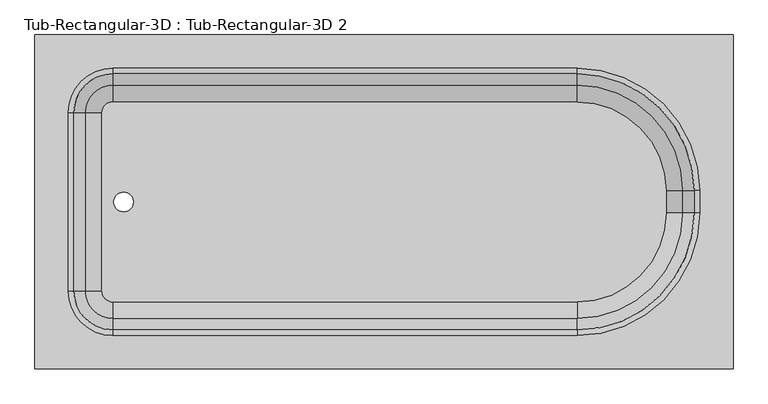
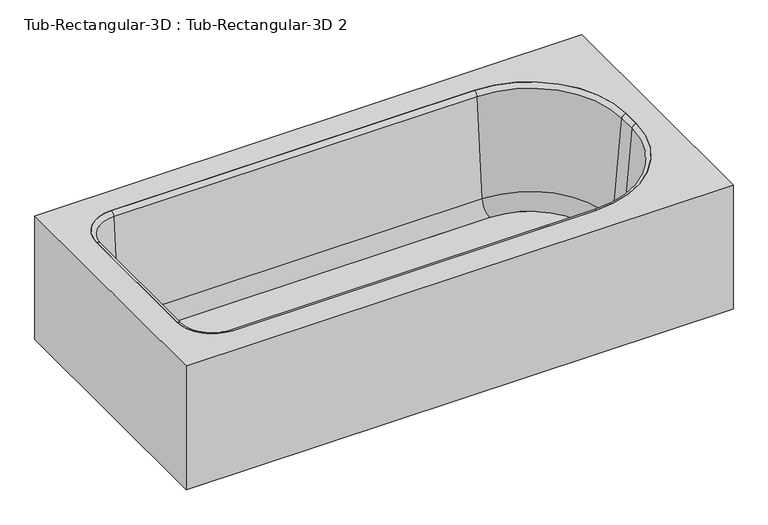
"""IFC4 building model written with IfcOpenShell, lengths in millimetres: flow terminal geometry, Tub-Rectangular-3D : Tub-Rectangular-3D 2."""

from ifc_helpers import new_model, si_unit, point, frame, frame_2d, origin, place, context, project, spatial, polyline, circle_curve, ellipse_curve, trimmed, segment, composite_curve, outline, extrude, source, transform, mapped, element, save
from ifc_brep_helpers import plane_surface, cylinder_surface, revolved_surface, advanced_brep


def tub_rectangular_3d_tub_rectangular_3d_2_b18e5bc2(model_context):
    return source(origin(), model_context, "Body", "SolidModel", [
        advanced_brep(
        [(480.0720313, 830.2625, 381.0), (-1110.6029687, 830.2625, 381.0), (-1110.6029687, 68.2625, 381.0), (480.0720313, 68.2625, 381.0), (-932.8029687, 754.0625, 381.0), (124.4720313, 754.0625, 381.0), (403.8720313, 474.6625, 381.0), (403.8720313, 423.8625, 381.0), (124.4720313, 144.4625, 381.0), (-932.8029687, 144.4625, 381.0), (-1034.4029687, 246.0625, 381.0), (-1034.4029687, 652.4625, 381.0), (461.0220313, 811.2125, 361.95), (461.0220313, 87.3125, 361.95), (-1091.5529687, 87.3125, 361.95), (-1091.5529687, 811.2125, 361.95), (-932.8029687, 754.0625, 361.95), (-1034.4029687, 652.4625, 361.95), (-1034.4029687, 246.0625, 361.95), (-932.8029687, 144.4625, 361.95), (124.4720313, 144.4625, 361.95), (403.8720313, 423.8625, 361.95), (403.8720313, 474.6625, 361.95), (124.4720313, 754.0625, 361.95), (480.0720313, 830.2625, 0.0), (-1110.6029687, 830.2625, 0.0), (-1110.6029687, 68.2625, 0.0), (480.0720313, 68.2625, 0.0), (461.0220313, 811.2125, 0.0), (-1091.5529687, 811.2125, 0.0), (-1091.5529687, 87.3125, 0.0), (461.0220313, 87.3125, 0.0)],
        [
            (0, 1),
            (1, 2),
            (2, 3),
            (3, 0),
            (4, 5),
            (5, 6, circle_curve(frame((124.4720313, 474.6625, 381.0), z_axis=(0.0, 0.0, -1.0), x_axis=(0.0, 1.0, 0.0)), 279.4)),
            (6, 7),
            (7, 8, circle_curve(frame((124.4720313, 423.8625, 381.0), z_axis=(0.0, 0.0, -1.0), x_axis=(0.0, 1.0, 0.0)), 279.4)),
            (8, 9),
            (9, 10, circle_curve(frame((-932.8029687, 246.0625, 381.0), z_axis=(0.0, 0.0, -1.0), x_axis=(0.0, 1.0, 0.0)), 101.6)),
            (10, 11),
            (11, 4, circle_curve(frame((-932.8029687, 652.4625, 381.0), z_axis=(0.0, 0.0, -1.0), x_axis=(0.0, 1.0, 0.0)), 101.6)),
            (12, 13),
            (13, 14),
            (14, 15),
            (15, 12),
            (16, 17, circle_curve(frame((-932.8029687, 652.4625, 361.95), z_axis=(0.0, 0.0, 1.0), x_axis=(0.0, 1.0, 0.0)), 101.6)),
            (17, 18),
            (18, 19, circle_curve(frame((-932.8029687, 246.0625, 361.95), z_axis=(0.0, 0.0, 1.0), x_axis=(0.0, 1.0, 0.0)), 101.6)),
            (19, 20),
            (20, 21, circle_curve(frame((124.4720313, 423.8625, 361.95), z_axis=(0.0, 0.0, 1.0), x_axis=(0.0, 1.0, 0.0)), 279.4)),
            (21, 22),
            (22, 23, circle_curve(frame((124.4720313, 474.6625, 361.95), z_axis=(0.0, 0.0, 1.0), x_axis=(0.0, 1.0, 0.0)), 279.4)),
            (23, 16),
            (0, 24),
            (24, 25),
            (25, 1),
            (25, 26),
            (26, 2),
            (26, 27),
            (27, 3),
            (27, 24),
            (4, 16),
            (23, 5),
            (22, 6),
            (21, 7),
            (20, 8),
            (19, 9),
            (18, 10),
            (17, 11),
            (28, 29),
            (29, 30),
            (30, 31),
            (31, 28),
            (31, 13),
            (12, 28),
            (30, 14),
            (29, 15),
        ],
        [
            plane_surface(frame((-1110.6029687, 830.2625, 381.0), z_axis=(0.0, 0.0, 1.0), x_axis=(-1.0, 0.0, 0.0))),
            plane_surface(frame((-1110.6029687, 830.2625, 361.95), z_axis=(0.0, 0.0, -1.0), x_axis=(1.0, 0.0, 0.0))),
            plane_surface(frame((480.0720313, 830.2625, 381.0), z_axis=(0.0, 1.0, 0.0), x_axis=(0.0, 0.0, -1.0))),
            plane_surface(frame((-1110.6029687, 830.2625, 381.0), z_axis=(-1.0, 0.0, 0.0), x_axis=(0.0, 0.0, -1.0))),
            plane_surface(frame((-1110.6029687, 68.2625, 381.0), z_axis=(0.0, -1.0, 0.0), x_axis=(0.0, 0.0, -1.0))),
            plane_surface(frame((480.0720313, 68.2625, 381.0), z_axis=(1.0, 0.0, 0.0), x_axis=(0.0, 0.0, -1.0))),
            plane_surface(frame((-932.8029687, 754.0625, 381.0), z_axis=(0.0, -1.0, 0.0), x_axis=(0.0, 0.0, -1.0))),
            revolved_surface(polyline([(124.4720313, 754.0625, 361.95), (124.4720313, 754.0625, 381.0)]), (124.4720313, 474.6625, 381.0), (0.0, 0.0, -1.0)),
            plane_surface(frame((403.8720313, 474.6625, 381.0), z_axis=(-1.0, 0.0, 0.0), x_axis=(0.0, 0.0, -1.0))),
            revolved_surface(polyline([(124.4720313, 703.2625, 361.95), (124.4720313, 703.2625, 381.0)]), (124.4720313, 423.8625, 381.0), (0.0, 0.0, -1.0)),
            plane_surface(frame((124.4720313, 144.4625, 381.0), z_axis=(0.0, 1.0, 0.0), x_axis=(0.0, 0.0, -1.0))),
            revolved_surface(polyline([(-932.8029687, 347.6625, 361.95), (-932.8029687, 347.6625, 381.0)]), (-932.8029687, 246.0625, 381.0), (0.0, 0.0, -1.0)),
            plane_surface(frame((-1034.4029687, 246.0625, 381.0), z_axis=(1.0, 0.0, 0.0), x_axis=(0.0, 0.0, -1.0))),
            revolved_surface(polyline([(-932.8029687, 754.0625, 361.95), (-932.8029687, 754.0625, 381.0)]), (-932.8029687, 652.4625, 381.0), (0.0, 0.0, -1.0)),
            plane_surface(frame((-1110.6029687, 830.2625, 0.0), z_axis=(0.0, 0.0, -1.0), x_axis=(1.0, 0.0, 0.0))),
            plane_surface(frame((461.0220313, 811.2125, 361.95), z_axis=(-1.0, 0.0, 0.0), x_axis=(0.0, 0.0, -1.0))),
            plane_surface(frame((461.0220313, 87.3125, 361.95), z_axis=(0.0, 1.0, 0.0), x_axis=(0.0, 0.0, -1.0))),
            plane_surface(frame((-1091.5529687, 87.3125, 361.95), z_axis=(1.0, 0.0, 0.0), x_axis=(0.0, 0.0, -1.0))),
            plane_surface(frame((-1091.5529687, 811.2125, 361.95), z_axis=(0.0, -1.0, 0.0), x_axis=(0.0, 0.0, -1.0))),
        ],
        [
            (0, [[1, 2, 3, 4], [5, 6, 7, 8, 9, 10, 11, 12]]),
            (1, [[13, 14, 15, 16], [17, 18, 19, 20, 21, 22, 23, 24]]),
            (2, [[-1, 25, 26, 27]]),
            (3, [[-2, -27, 28, 29]]),
            (4, [[-3, -29, 30, 31]]),
            (5, [[-25, -4, -31, 32]]),
            (6, [[-5, 33, -24, 34]]),
            (7, [[-6, -34, -23, 35]]),
            (8, [[-7, -35, -22, 36]]),
            (9, [[-8, -36, -21, 37]]),
            (10, [[-9, -37, -20, 38]]),
            (11, [[-10, -38, -19, 39]]),
            (12, [[-11, -39, -18, 40]]),
            (13, [[-12, -40, -17, -33]]),
            (14, [[-32, -30, -28, -26], [41, 42, 43, 44]]),
            (15, [[-44, 45, -13, 46]]),
            (16, [[-43, 47, -14, -45]]),
            (17, [[-42, 48, -15, -47]]),
            (18, [[-41, -46, -16, -48]]),
        ],
    ),
        extrude(outline(composite_curve([segment(trimmed(circle_curve(frame_2d((124.4720313, 474.6625)), 202.7964741), [point((124.4720313, 677.4589741))], [point((327.2685054, 474.6625))], False, "CARTESIAN"), True, "CONTINUOUS"), segment(polyline([(327.2685054, 474.6625), (327.2685054, 423.8625)]), True, "CONTINUOUS"), segment(trimmed(circle_curve(frame_2d((124.4720313, 423.8625)), 202.7964741), [point((327.2685054, 423.8625))], [point((124.4720313, 221.0660259))], False, "CARTESIAN"), True, "CONTINUOUS"), segment(polyline([(124.4720313, 221.0660259), (-932.8029687, 221.0660259)]), True, "CONTINUOUS"), segment(trimmed(circle_curve(frame_2d((-932.8029687, 246.0625)), 24.9964741), [point((-932.8029687, 221.0660259))], [point((-957.7994428, 246.0625))], False, "CARTESIAN"), True, "CONTINUOUS"), segment(polyline([(-957.7994428, 246.0625), (-957.7994428, 652.4625)]), True, "CONTINUOUS"), segment(trimmed(circle_curve(frame_2d((-932.8029687, 652.4625)), 24.9964741), [point((-957.7994428, 652.4625))], [point((-932.8029687, 677.4589741))], False, "CARTESIAN"), True, "CONTINUOUS"), segment(polyline([(-932.8029687, 677.4589741), (124.4720313, 677.4589741)]), True, "CONTINUOUS")], self_intersect=False), holes=[composite_curve([segment(trimmed(circle_curve(frame_2d((-908.510206, 449.2625)), 22.225), [point((-908.510206, 471.4875))], [point((-908.510206, 427.0375))], True, "CARTESIAN"), True, "CONTINUOUS"), segment(trimmed(circle_curve(frame_2d((-908.510206, 449.2625)), 22.225), [point((-908.510206, 427.0375))], [point((-908.510206, 471.4875))], True, "CARTESIAN"), True, "CONTINUOUS")], self_intersect=False)]), frame((0.0, 0.0, 16.863573), z_axis=(0.0, 0.0, 1.0), x_axis=(1.0, 0.0, 0.0)), (0.0, 0.0, 1.0), 19.05),
        advanced_brep(
        [(-995.7544608, 652.4625, 70.6929392), (-932.8029687, 715.4139921, 70.6929392), (-932.8029687, 741.5845035, 369.8232535), (-1021.9249722, 652.4625, 369.8232535), (-957.7994428, 652.4625, 35.913573), (-932.8029687, 677.4589741, 35.913573), (-957.7994428, 652.4625, 16.863573), (-932.8029687, 677.4589741, 16.863573), (-1034.4029687, 652.4625, 16.863573), (-932.8029687, 754.0625, 16.863573), (-1034.4029687, 652.4625, 381.0), (-932.8029687, 754.0625, 381.0), (-1021.9249722, 246.0625, 369.8232535), (-995.7544608, 246.0625, 70.6929392), (-957.7994428, 246.0625, 35.913573), (-957.7994428, 246.0625, 16.863573), (-1034.4029687, 246.0625, 16.863573), (-1034.4029687, 246.0625, 381.0), (-932.8029687, 183.1110079, 70.6929392), (-932.8029687, 156.9404965, 369.8232535), (-932.8029687, 221.0660259, 35.913573), (-932.8029687, 221.0660259, 16.863573), (-932.8029687, 144.4625, 16.863573), (-932.8029687, 144.4625, 381.0), (124.4720313, 156.9404965, 369.8232535), (124.4720313, 183.1110079, 70.6929392), (124.4720313, 221.0660259, 35.913573), (124.4720313, 221.0660259, 16.863573), (124.4720313, 144.4625, 16.863573), (124.4720313, 144.4625, 381.0), (365.2235234, 423.8625, 70.6929392), (391.3940348, 423.8625, 369.8232535), (327.2685054, 423.8625, 35.913573), (327.2685054, 423.8625, 16.863573), (403.8720313, 423.8625, 16.863573), (403.8720313, 423.8625, 381.0), (391.3940348, 474.6625, 369.8232535), (365.2235234, 474.6625, 70.6929392), (327.2685054, 474.6625, 35.913573), (327.2685054, 474.6625, 16.863573), (403.8720313, 474.6625, 16.863573), (403.8720313, 474.6625, 381.0), (124.4720313, 715.4139921, 70.6929392), (124.4720313, 741.5845035, 369.8232535), (124.4720313, 677.4589741, 35.913573), (124.4720313, 677.4589741, 16.863573), (124.4720313, 754.0625, 16.863573), (124.4720313, 754.0625, 381.0)],
        [
            (0, 1, circle_curve(frame((-932.8029687, 652.4625, 70.6929392), z_axis=(0.0, 0.0, -1.0), x_axis=(0.0, 1.0, 0.0)), 62.9514921)),
            (1, 2),
            (2, 3, circle_curve(frame((-932.8029687, 652.4625, 369.8232535), z_axis=(0.0, 0.0, 1.0), x_axis=(0.0, 1.0, 0.0)), 89.1220035)),
            (3, 0),
            (4, 5, circle_curve(frame((-932.8029687, 652.4625, 35.913573), z_axis=(0.0, 0.0, -1.0), x_axis=(0.0, 1.0, 0.0)), 24.9964741)),
            (5, 1, circle_curve(frame((-932.8029687, 677.4589741, 74.013573), z_axis=(1.0, 0.0, 0.0), x_axis=(0.0, -1.0, 0.0)), 38.1)),
            (0, 4, circle_curve(frame((-957.7994428, 652.4625, 74.013573), z_axis=(0.0, -1.0, 0.0), x_axis=(1.0, 0.0, 0.0)), 38.1)),
            (6, 7, circle_curve(frame((-932.8029687, 652.4625, 16.863573), z_axis=(0.0, 0.0, -1.0), x_axis=(0.0, 1.0, 0.0)), 24.9964741)),
            (7, 5),
            (4, 6),
            (8, 9, circle_curve(frame((-932.8029687, 652.4625, 16.863573), z_axis=(0.0, 0.0, -1.0), x_axis=(0.0, 1.0, 0.0)), 101.6)),
            (9, 7),
            (6, 8),
            (10, 11, circle_curve(frame((-932.8029687, 652.4625, 381.0), z_axis=(0.0, 0.0, -1.0), x_axis=(0.0, 1.0, 0.0)), 101.6)),
            (11, 9),
            (8, 10),
            (2, 11, circle_curve(frame((-932.8029687, 754.0625, 368.4462547), z_axis=(-1.0, 0.0, 0.0), x_axis=(0.0, -1.0, 0.0)), 12.5537453)),
            (10, 3, circle_curve(frame((-1034.4029687, 652.4625, 368.4462547), z_axis=(0.0, 1.0, 0.0), x_axis=(1.0, 0.0, 0.0)), 12.5537453)),
            (3, 12),
            (12, 13),
            (13, 0),
            (13, 14, circle_curve(frame((-957.7994428, 246.0625, 74.013573), z_axis=(0.0, -1.0, 0.0), x_axis=(1.0, 0.0, 0.0)), 38.1)),
            (14, 4),
            (14, 15),
            (15, 6),
            (15, 16),
            (16, 8),
            (16, 17),
            (17, 10),
            (17, 12, circle_curve(frame((-1034.4029687, 246.0625, 368.4462547), z_axis=(0.0, 1.0, 0.0), x_axis=(1.0, 0.0, 0.0)), 12.5537453)),
            (18, 13, circle_curve(frame((-932.8029687, 246.0625, 70.6929392), z_axis=(0.0, 0.0, -1.0), x_axis=(-1.0, 0.0, 0.0)), 62.9514921)),
            (12, 19, circle_curve(frame((-932.8029687, 246.0625, 369.8232535), z_axis=(0.0, 0.0, 1.0), x_axis=(-1.0, 0.0, 0.0)), 89.1220035)),
            (19, 18),
            (20, 14, circle_curve(frame((-932.8029687, 246.0625, 35.913573), z_axis=(0.0, 0.0, -1.0), x_axis=(-1.0, 0.0, 0.0)), 24.9964741)),
            (18, 20, circle_curve(frame((-932.8029687, 221.0660259, 74.013573), z_axis=(1.0, 0.0, 0.0), x_axis=(0.0, 1.0, 0.0)), 38.1)),
            (21, 15, circle_curve(frame((-932.8029687, 246.0625, 16.863573), z_axis=(0.0, 0.0, -1.0), x_axis=(-1.0, 0.0, 0.0)), 24.9964741)),
            (20, 21),
            (22, 16, circle_curve(frame((-932.8029687, 246.0625, 16.863573), z_axis=(0.0, 0.0, -1.0), x_axis=(-1.0, 0.0, 0.0)), 101.6)),
            (21, 22),
            (23, 17, circle_curve(frame((-932.8029687, 246.0625, 381.0), z_axis=(0.0, 0.0, -1.0), x_axis=(-1.0, 0.0, 0.0)), 101.6)),
            (22, 23),
            (23, 19, circle_curve(frame((-932.8029687, 144.4625, 368.4462547), z_axis=(-1.0, 0.0, 0.0), x_axis=(0.0, 1.0, 0.0)), 12.5537453)),
            (19, 24),
            (24, 25),
            (25, 18),
            (25, 26, circle_curve(frame((124.4720313, 221.0660259, 74.013573), z_axis=(1.0, 0.0, 0.0), x_axis=(0.0, 1.0, 0.0)), 38.1)),
            (26, 20),
            (26, 27),
            (27, 21),
            (27, 28),
            (28, 22),
            (28, 29),
            (29, 23),
            (29, 24, circle_curve(frame((124.4720313, 144.4625, 368.4462547), z_axis=(-1.0, 0.0, 0.0), x_axis=(0.0, 1.0, 0.0)), 12.5537453)),
            (30, 25, circle_curve(frame((124.4720313, 423.8625, 70.6929392), z_axis=(0.0, 0.0, -1.0), x_axis=(0.0, -1.0, 0.0)), 240.7514921)),
            (24, 31, circle_curve(frame((124.4720313, 423.8625, 369.8232535), z_axis=(0.0, 0.0, 1.0), x_axis=(0.0, -1.0, 0.0)), 266.9220035)),
            (31, 30),
            (32, 26, circle_curve(frame((124.4720313, 423.8625, 35.913573), z_axis=(0.0, 0.0, -1.0), x_axis=(0.0, -1.0, 0.0)), 202.7964741)),
            (30, 32, circle_curve(frame((327.2685054, 423.8625, 74.013573), z_axis=(0.0, 1.0, 0.0), x_axis=(-1.0, 0.0, 0.0)), 38.1)),
            (33, 27, circle_curve(frame((124.4720313, 423.8625, 16.863573), z_axis=(0.0, 0.0, -1.0), x_axis=(0.0, -1.0, 0.0)), 202.7964741)),
            (32, 33),
            (34, 28, circle_curve(frame((124.4720313, 423.8625, 16.863573), z_axis=(0.0, 0.0, -1.0), x_axis=(0.0, -1.0, 0.0)), 279.4)),
            (33, 34),
            (35, 29, circle_curve(frame((124.4720313, 423.8625, 381.0), z_axis=(0.0, 0.0, -1.0), x_axis=(0.0, -1.0, 0.0)), 279.4)),
            (34, 35),
            (35, 31, circle_curve(frame((403.8720313, 423.8625, 368.4462547), z_axis=(0.0, -1.0, 0.0), x_axis=(-1.0, 0.0, 0.0)), 12.5537453)),
            (31, 36),
            (36, 37),
            (37, 30),
            (37, 38, circle_curve(frame((327.2685054, 474.6625, 74.013573), z_axis=(0.0, 1.0, 0.0), x_axis=(-1.0, 0.0, 0.0)), 38.1)),
            (38, 32),
            (38, 39),
            (39, 33),
            (39, 40),
            (40, 34),
            (40, 41),
            (41, 35),
            (41, 36, circle_curve(frame((403.8720313, 474.6625, 368.4462547), z_axis=(0.0, -1.0, 0.0), x_axis=(-1.0, 0.0, 0.0)), 12.5537453)),
            (42, 37, circle_curve(frame((124.4720313, 474.6625, 70.6929392), z_axis=(0.0, 0.0, -1.0), x_axis=(1.0, 0.0, 0.0)), 240.7514921)),
            (36, 43, circle_curve(frame((124.4720313, 474.6625, 369.8232535), z_axis=(0.0, 0.0, 1.0), x_axis=(1.0, 0.0, 0.0)), 266.9220035)),
            (43, 42),
            (44, 38, circle_curve(frame((124.4720313, 474.6625, 35.913573), z_axis=(0.0, 0.0, -1.0), x_axis=(1.0, 0.0, 0.0)), 202.7964741)),
            (42, 44, circle_curve(frame((124.4720313, 677.4589741, 74.013573), z_axis=(-1.0, 0.0, 0.0), x_axis=(0.0, -1.0, 0.0)), 38.1)),
            (45, 39, circle_curve(frame((124.4720313, 474.6625, 16.863573), z_axis=(0.0, 0.0, -1.0), x_axis=(1.0, 0.0, 0.0)), 202.7964741)),
            (44, 45),
            (46, 40, circle_curve(frame((124.4720313, 474.6625, 16.863573), z_axis=(0.0, 0.0, -1.0), x_axis=(1.0, 0.0, 0.0)), 279.4)),
            (45, 46),
            (47, 41, circle_curve(frame((124.4720313, 474.6625, 381.0), z_axis=(0.0, 0.0, -1.0), x_axis=(1.0, 0.0, 0.0)), 279.4)),
            (46, 47),
            (47, 43, circle_curve(frame((124.4720313, 754.0625, 368.4462547), z_axis=(1.0, 0.0, 0.0), x_axis=(0.0, -1.0, 0.0)), 12.5537453)),
            (43, 2),
            (1, 42),
            (5, 44),
            (7, 45),
            (9, 46),
            (11, 47),
        ],
        [
            revolved_surface(polyline([(-932.8029687, 741.5845035, 369.8232535), (-932.8029687, 715.4139921, 70.6929392)]), (-932.8029687, 652.4625, 381.0), (0.0, 0.0, 1.0)),
            revolved_surface(trimmed(ellipse_curve(frame((-932.8029687, 677.4589741, 74.013573), z_axis=(-1.0, 0.0, 0.0), x_axis=(0.0, -1.0, 0.0)), 38.1, 38.1), [point((-932.8029687, 715.4139921, 70.6929392))], [point((-932.8029687, 677.4589741, 35.913573))], True, "CARTESIAN"), (-932.8029687, 652.4625, 381.0), (0.0, 0.0, 1.0)),
            revolved_surface(polyline([(-932.8029687, 677.4589741, 35.913572999999985), (-932.8029687, 677.4589741, 16.863572999999974)]), (-932.8029687, 652.4625, 381.0), (0.0, 0.0, 1.0)),
            plane_surface(frame((-932.8029687, 652.4625, 16.863573), z_axis=(0.0, 0.0, -1.0), x_axis=(0.0, 1.0, 0.0))),
            cylinder_surface(frame((-932.8029687, 652.4625, 381.0), z_axis=(0.0, 0.0, 1.0), x_axis=(0.0, 1.0, 0.0)), 101.6),
            revolved_surface(trimmed(ellipse_curve(frame((-932.8029687, 754.0625, 368.4462547), z_axis=(1.0, 0.0, 0.0), x_axis=(0.0, -1.0, 0.0)), 12.5537453, 12.5537453), [point((-932.8029687, 754.0625, 381.0))], [point((-932.8029687, 741.5845035, 369.8232535))], True, "CARTESIAN"), (-932.8029687, 652.4625, 381.0), (0.0, 0.0, 1.0)),
            plane_surface(frame((-1021.9249722, 652.4625, 369.8232535), z_axis=(0.9961946980917458, 0.0, 0.08715574274765595), x_axis=(0.0, -1.0, 0.0))),
            revolved_surface(polyline([(-919.6994427999999, 246.0625, 74.013573), (-919.6994427999999, 652.4625, 74.013573)]), (-957.7994428, 652.4625, 74.013573), (0.0, -1.0, 0.0)),
            plane_surface(frame((-957.7994428, 652.4625, 35.913573), z_axis=(1.0, 0.0, 0.0), x_axis=(0.0, -1.0, 0.0))),
            plane_surface(frame((-957.7994428, 652.4625, 16.863573), z_axis=(0.0, 0.0, -1.0), x_axis=(0.0, -1.0, 0.0))),
            plane_surface(frame((-1034.4029687, 652.4625, 16.863573), z_axis=(-1.0, 0.0, 0.0), x_axis=(0.0, -1.0, 0.0))),
            cylinder_surface(frame((-1034.4029687, 652.4625, 368.4462547), z_axis=(0.0, 1.0, 0.0), x_axis=(1.0, 0.0, 0.0)), 12.5537453),
            revolved_surface(polyline([(-1021.9249722, 246.0625, 369.8232535), (-995.7544608, 246.0625, 70.6929392)]), (-932.8029687, 246.0625, 381.0), (0.0, 0.0, 1.0)),
            revolved_surface(trimmed(ellipse_curve(frame((-957.7994428, 246.0625, 74.013573), z_axis=(0.0, -1.0, 0.0), x_axis=(1.0, 0.0, 0.0)), 38.1, 38.1), [point((-995.7544608, 246.0625, 70.6929392))], [point((-957.7994428, 246.0625, 35.913573))], True, "CARTESIAN"), (-932.8029687, 246.0625, 381.0), (0.0, 0.0, 1.0)),
            revolved_surface(polyline([(-957.7994428, 246.0625, 35.913572999999985), (-957.7994428, 246.0625, 16.863572999999974)]), (-932.8029687, 246.0625, 381.0), (0.0, 0.0, 1.0)),
            plane_surface(frame((-932.8029687, 246.0625, 16.863573), z_axis=(0.0, 0.0, -1.0), x_axis=(-1.0, 0.0, 0.0))),
            cylinder_surface(frame((-932.8029687, 246.0625, 381.0), z_axis=(0.0, 0.0, 1.0), x_axis=(-1.0, 0.0, 0.0)), 101.6),
            revolved_surface(trimmed(ellipse_curve(frame((-1034.4029687, 246.0625, 368.4462547), z_axis=(0.0, 1.0, 0.0), x_axis=(1.0, 0.0, 0.0)), 12.5537453, 12.5537453), [point((-1034.4029687, 246.0625, 381.0))], [point((-1021.9249722, 246.0625, 369.8232535))], True, "CARTESIAN"), (-932.8029687, 246.0625, 381.0), (0.0, 0.0, 1.0)),
            plane_surface(frame((-932.8029687, 156.9404965, 369.8232535), z_axis=(0.0, 0.9961946980917461, 0.08715574274765271), x_axis=(1.0, 0.0, 0.0))),
            revolved_surface(polyline([(124.47203129999991, 259.1660259, 74.013573), (-932.8029687, 259.1660259, 74.013573)]), (-932.8029687, 221.0660259, 74.013573), (1.0, 0.0, 0.0)),
            plane_surface(frame((-932.8029687, 221.0660259, 35.913573), z_axis=(0.0, 1.0, 0.0), x_axis=(1.0, 0.0, 0.0))),
            plane_surface(frame((-932.8029687, 221.0660259, 16.863573), z_axis=(0.0, 0.0, -1.0), x_axis=(1.0, 0.0, 0.0))),
            plane_surface(frame((-932.8029687, 144.4625, 16.863573), z_axis=(0.0, -1.0, 0.0), x_axis=(1.0, 0.0, 0.0))),
            cylinder_surface(frame((-932.8029687, 144.4625, 368.4462547), z_axis=(-1.0, 0.0, 0.0), x_axis=(0.0, 1.0, 0.0)), 12.5537453),
            revolved_surface(polyline([(124.4720313, 156.9404965, 369.8232535), (124.4720313, 183.1110079, 70.6929392)]), (124.4720313, 423.8625, 381.0), (0.0, 0.0, 1.0)),
            revolved_surface(trimmed(ellipse_curve(frame((124.4720313, 221.0660259, 74.013573), z_axis=(1.0, 0.0, 0.0), x_axis=(0.0, 1.0, 0.0)), 38.1, 38.1), [point((124.4720313, 183.1110079, 70.6929392))], [point((124.4720313, 221.0660259, 35.913573))], True, "CARTESIAN"), (124.4720313, 423.8625, 381.0), (0.0, 0.0, 1.0)),
            revolved_surface(polyline([(124.4720313, 221.0660259, 35.913572999999985), (124.4720313, 221.0660259, 16.863572999999974)]), (124.4720313, 423.8625, 381.0), (0.0, 0.0, 1.0)),
            plane_surface(frame((124.4720313, 423.8625, 16.863573), z_axis=(0.0, 0.0, -1.0), x_axis=(0.0, -1.0, 0.0))),
            cylinder_surface(frame((124.4720313, 423.8625, 381.0), z_axis=(0.0, 0.0, 1.0), x_axis=(0.0, -1.0, 0.0)), 279.4),
            revolved_surface(trimmed(ellipse_curve(frame((124.4720313, 144.4625, 368.4462547), z_axis=(-1.0, 0.0, 0.0), x_axis=(0.0, 1.0, 0.0)), 12.5537453, 12.5537453), [point((124.4720313, 144.4625, 381.0))], [point((124.4720313, 156.9404965, 369.8232535))], True, "CARTESIAN"), (124.4720313, 423.8625, 381.0), (0.0, 0.0, 1.0)),
            plane_surface(frame((391.3940348, 423.8625, 369.8232535), z_axis=(-0.9961946980917464, 0.0, 0.08715574274764948), x_axis=(0.0, 1.0, 0.0))),
            revolved_surface(polyline([(289.16850539999996, 474.6625, 74.013573), (289.16850539999996, 423.8625, 74.013573)]), (327.2685054, 423.8625, 74.013573), (0.0, 1.0, 0.0)),
            plane_surface(frame((327.2685054, 423.8625, 35.913573), z_axis=(-1.0, 0.0, 0.0), x_axis=(0.0, 1.0, 0.0))),
            plane_surface(frame((327.2685054, 423.8625, 16.863573), z_axis=(0.0, 0.0, -1.0), x_axis=(0.0, 1.0, 0.0))),
            plane_surface(frame((403.8720313, 423.8625, 16.863573), z_axis=(1.0, 0.0, 0.0), x_axis=(0.0, 1.0, 0.0))),
            cylinder_surface(frame((403.8720313, 423.8625, 368.4462547), z_axis=(0.0, -1.0, 0.0), x_axis=(-1.0, 0.0, 0.0)), 12.5537453),
            revolved_surface(polyline([(391.3940348, 474.6625, 369.8232535), (365.2235234, 474.6625, 70.6929392)]), (124.4720313, 474.6625, 381.0), (0.0, 0.0, 1.0)),
            revolved_surface(trimmed(ellipse_curve(frame((327.2685054, 474.6625, 74.013573), z_axis=(0.0, 1.0, 0.0), x_axis=(-1.0, 0.0, 0.0)), 38.1, 38.1), [point((365.2235234, 474.6625, 70.6929392))], [point((327.2685054, 474.6625, 35.913573))], True, "CARTESIAN"), (124.4720313, 474.6625, 381.0), (0.0, 0.0, 1.0)),
            revolved_surface(polyline([(327.2685054, 474.6625, 35.913572999999985), (327.2685054, 474.6625, 16.863572999999974)]), (124.4720313, 474.6625, 381.0), (0.0, 0.0, 1.0)),
            plane_surface(frame((124.4720313, 474.6625, 16.863573), z_axis=(0.0, 0.0, -1.0), x_axis=(1.0, 0.0, 0.0))),
            cylinder_surface(frame((124.4720313, 474.6625, 381.0), z_axis=(0.0, 0.0, 1.0), x_axis=(1.0, 0.0, 0.0)), 279.4),
            revolved_surface(trimmed(ellipse_curve(frame((403.8720313, 474.6625, 368.4462547), z_axis=(0.0, -1.0, 0.0), x_axis=(-1.0, 0.0, 0.0)), 12.5537453, 12.5537453), [point((403.8720313, 474.6625, 381.0))], [point((391.3940348, 474.6625, 369.8232535))], True, "CARTESIAN"), (124.4720313, 474.6625, 381.0), (0.0, 0.0, 1.0)),
            plane_surface(frame((124.4720313, 741.5845035, 369.8232535), z_axis=(0.0, -0.9961946980917461, 0.08715574274765271), x_axis=(-1.0, 0.0, 0.0))),
            revolved_surface(polyline([(-932.8029686999998, 639.3589741, 74.013573), (124.4720313, 639.3589741, 74.013573)]), (124.4720313, 677.4589741, 74.013573), (-1.0, 0.0, 0.0)),
            plane_surface(frame((124.4720313, 677.4589741, 35.913573), z_axis=(0.0, -1.0, 0.0), x_axis=(-1.0, 0.0, 0.0))),
            plane_surface(frame((124.4720313, 677.4589741, 16.863573), z_axis=(0.0, 0.0, -1.0), x_axis=(-1.0, 0.0, 0.0))),
            plane_surface(frame((124.4720313, 754.0625, 16.863573), z_axis=(0.0, 1.0, 0.0), x_axis=(-1.0, 0.0, 0.0))),
            cylinder_surface(frame((124.4720313, 754.0625, 368.4462547), z_axis=(1.0, 0.0, 0.0), x_axis=(0.0, -1.0, 0.0)), 12.5537453),
        ],
        [
            (0, [[1, 2, 3, 4]]),
            (1, [[5, 6, -1, 7]]),
            (2, [[8, 9, -5, 10]]),
            (3, [[11, 12, -8, 13]]),
            (4, [[14, 15, -11, 16]]),
            (5, [[-3, 17, -14, 18]]),
            (6, [[-4, 19, 20, 21]]),
            (7, [[-7, -21, 22, 23]]),
            (8, [[-10, -23, 24, 25]]),
            (9, [[-13, -25, 26, 27]]),
            (10, [[-16, -27, 28, 29]]),
            (11, [[-18, -29, 30, -19]]),
            (12, [[31, -20, 32, 33]]),
            (13, [[34, -22, -31, 35]]),
            (14, [[36, -24, -34, 37]]),
            (15, [[38, -26, -36, 39]]),
            (16, [[40, -28, -38, 41]]),
            (17, [[-32, -30, -40, 42]]),
            (18, [[-33, 43, 44, 45]]),
            (19, [[-35, -45, 46, 47]]),
            (20, [[-37, -47, 48, 49]]),
            (21, [[-39, -49, 50, 51]]),
            (22, [[-41, -51, 52, 53]]),
            (23, [[-42, -53, 54, -43]]),
            (24, [[55, -44, 56, 57]]),
            (25, [[58, -46, -55, 59]]),
            (26, [[60, -48, -58, 61]]),
            (27, [[62, -50, -60, 63]]),
            (28, [[64, -52, -62, 65]]),
            (29, [[-56, -54, -64, 66]]),
            (30, [[-57, 67, 68, 69]]),
            (31, [[-59, -69, 70, 71]]),
            (32, [[-61, -71, 72, 73]]),
            (33, [[-63, -73, 74, 75]]),
            (34, [[-65, -75, 76, 77]]),
            (35, [[-66, -77, 78, -67]]),
            (36, [[79, -68, 80, 81]]),
            (37, [[82, -70, -79, 83]]),
            (38, [[84, -72, -82, 85]]),
            (39, [[86, -74, -84, 87]]),
            (40, [[88, -76, -86, 89]]),
            (41, [[-80, -78, -88, 90]]),
            (42, [[-81, 91, -2, 92]]),
            (43, [[-83, -92, -6, 93]]),
            (44, [[-85, -93, -9, 94]]),
            (45, [[-87, -94, -12, 95]]),
            (46, [[-89, -95, -15, 96]]),
            (47, [[-90, -96, -17, -91]]),
        ],
    ),
    ])


if __name__ == "__main__":
    model = new_model("IFC4")
    model_context = context("Model", 3, world=origin())
    ifc_project = project(units=[si_unit("LENGTHUNIT", "METRE", prefix="MILLI")], contexts=[model_context])
    site = spatial("IfcSite", under=ifc_project)
    building = spatial("IfcBuilding", under=site)
    placement = place(None, origin())
    tub_rectangular_3d_tub_rectangular_3d_2_shape = tub_rectangular_3d_tub_rectangular_3d_2_b18e5bc2(model_context)
    element("IfcFlowTerminal", 1, ObjectType="Tub-Rectangular-3D : Tub-Rectangular-3D 2", at=placement, inside=building, context=model_context, shape_type="MappedRepresentation", body=[
        mapped(tub_rectangular_3d_tub_rectangular_3d_2_shape, transform((0.0, 0.0, 0.0), x_axis=(1.0, 0.0, 0.0), y_axis=(0.0, 1.0, 0.0), z_axis=(0.0, 0.0, 1.0))),
    ])
    save(model, "model.ifc")

# Revit data of these elements
# Type "Tub-Rectangular-3D : Tub-Rectangular-3D 2"
#   Assembly Code = "D2010500"
#   Depth = 2' - 6"
#   Height = 1' - 3"
#   Width = 5' - 2 5/8"
#   Tub Material = Porcelain, Ivory
# Element 1 (IfcFlowTerminal, "Tub-Rectangular-3D : Tub-Rectangular-3D 2")
#   Materials on its faces: "Porcelain, Ivory"
# Materials
#   "Porcelain, Ivory": class "Ceramic", colour RGB 247 247 239, transparency 0, Description = "Porcelain, ivory", Cost = 0
